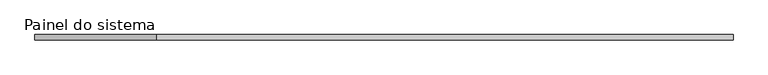
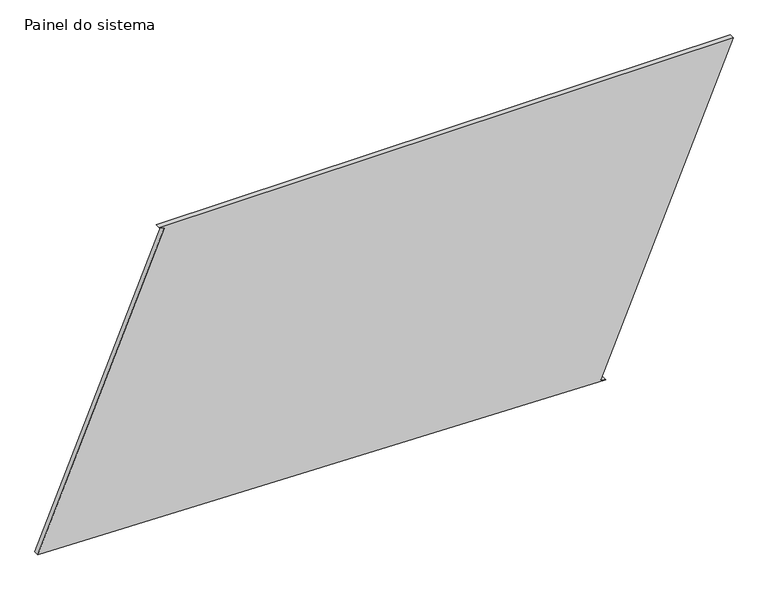
"""IFC4 building model written with IfcOpenShell, lengths in millimetres: plate geometry, Painel do sistema : Envidraçado."""

from ifc_helpers import new_model, si_unit, frame, origin, place, context, project, spatial, polyline, outline, extrude, source, transform, mapped, element, save


def painel_do_sistema_5ba6b536(model_context):
    return source(origin(), model_context, "Body", "SweptSolid", [
        extrude(outline(polyline([(0.0, 1060.557746), (9.6723918, 1037.5046586), (1526.0849425, 1673.7463932), (1526.0849425, -1089.0385837), (1516.4125507, -1065.9854964), (67.8809602, -1673.7463932), (0.0, 1060.557746)])), frame((0.0, 24.5, 0.0), z_axis=(0.0, 1.0, 0.0), x_axis=(0.0, 0.0, 1.0)), (0.0, 0.0, 1.0), 25.0),
    ])


if __name__ == "__main__":
    model = new_model("IFC4")
    model_context = context("Model", 3, world=origin())
    ifc_project = project(units=[si_unit("LENGTHUNIT", "METRE", prefix="MILLI")], contexts=[model_context])
    site = spatial("IfcSite", under=ifc_project)
    building = spatial("IfcBuilding", under=site)
    placement = place(None, origin())
    painel_do_sistema_shape = painel_do_sistema_5ba6b536(model_context)
    element("IfcPlate", 1, ObjectType="Painel do sistema : Envidraçado", at=placement, inside=building, context=model_context, shape_type="MappedRepresentation", body=[
        mapped(painel_do_sistema_shape, transform((0.0, 0.0, 0.0), x_axis=(1.0, 0.0, 0.0), y_axis=(0.0, 1.0, 0.0), z_axis=(0.0, 0.0, 1.0))),
    ])
    save(model, "model.ifc")

# Revit data of these elements
# Type "Painel do sistema : Envidraçado"
#   Construction Type Id = "GSP4R"
#   Analytic Construction = "Vidraça única Pilkington 1/8 pol"
#   Visual Light Transmittance = 0.9
#   Solar Heat Gain Coefficient = 0.86
#   Heat Transfer Coefficient (U) = 6.7069 W/(m²·K)
# Element 1 (IfcPlate, "Painel do sistema : Envidraçado")
#   Materials on its faces: "Vidro"
# Materials
#   "Vidro": class "Vidro", colour RGB 0 128 192, transparency 0.9, Description = "Vidro de sílica", Cost = 0
